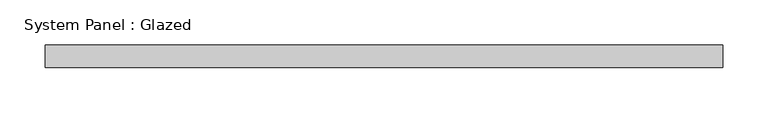
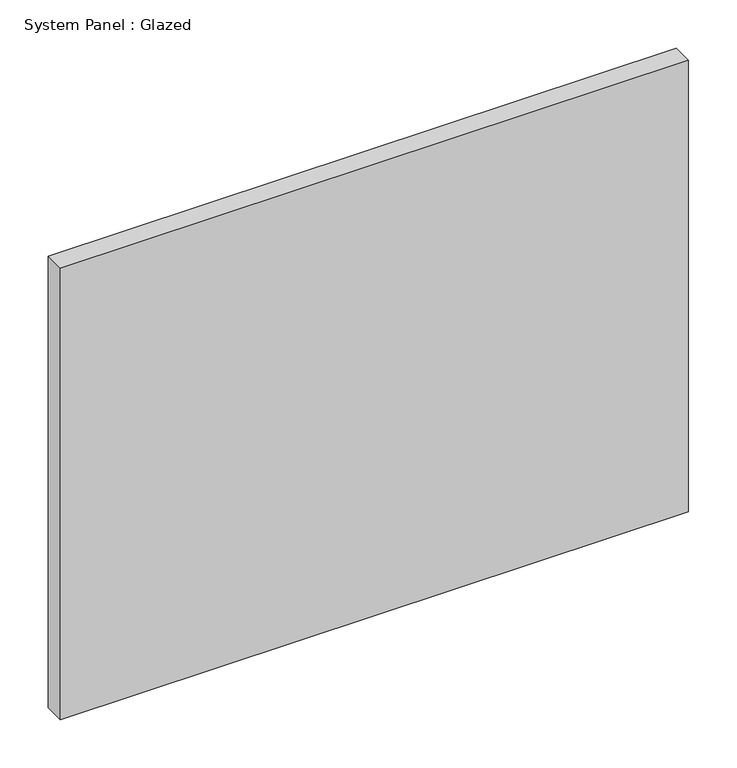
"""IFC4 building model written with IfcOpenShell, lengths in millimetres: plate geometry, System Panel : Glazed."""

from ifc_helpers import new_model, si_unit, origin, origin_with_axes, place, context, project, spatial, polyline, outline, extrude, source, transform, mapped, element, save


def system_panel_glazed_9f0f34b9(model_context):
    return source(origin(), model_context, "Body", "SweptSolid", [
        extrude(outline(polyline([(375.9636197, 19.05), (-375.9636197, 19.05), (-375.9636197, 44.45), (375.9636197, 44.45), (375.9636197, 19.05)])), origin_with_axes(), (0.0, 0.0, 1.0), 571.5),
    ])


if __name__ == "__main__":
    model = new_model("IFC4")
    model_context = context("Model", 3, world=origin())
    ifc_project = project(units=[si_unit("LENGTHUNIT", "METRE", prefix="MILLI")], contexts=[model_context])
    site = spatial("IfcSite", under=ifc_project)
    building = spatial("IfcBuilding", under=site)
    placement = place(None, origin())
    system_panel_glazed_shape = system_panel_glazed_9f0f34b9(model_context)
    element("IfcPlate", 1, ObjectType="System Panel : Glazed", at=placement, inside=building, context=model_context, shape_type="MappedRepresentation", body=[
        mapped(system_panel_glazed_shape, transform((0.0, 0.0, 0.0), x_axis=(1.0, 0.0, 0.0), y_axis=(0.0, 1.0, 0.0), z_axis=(0.0, 0.0, 1.0))),
    ])
    save(model, "model.ifc")

# Revit data of these elements
# Type "System Panel : Glazed"
#   Construction Type Id = "GSP4R"
#   Analytic Construction = "1/8 in Pilkington single glazing"
#   Visual Light Transmittance = 0.9
#   Solar Heat Gain Coefficient = 0.86
#   Heat Transfer Coefficient (U) = 1.18115 BTU/(h·ft²·°F)
#   Define Thermal Properties by = 1
# Element 1 (IfcPlate, "System Panel : Glazed")
#   Materials on its faces: "Glass"
# Materials
#   "Glass": class "Glass", colour RGB 0 128 192, transparency 0.75, Description = "Soda Lime Glass", Cost = 0
